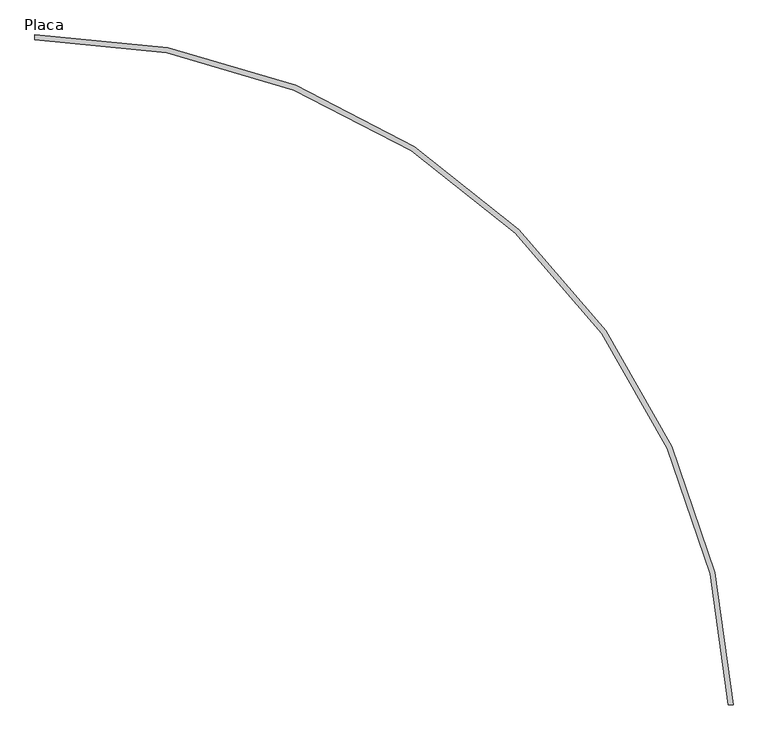
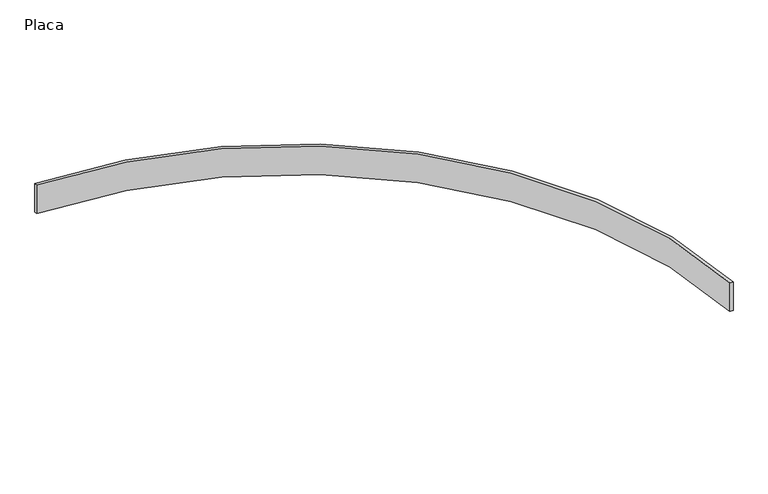
"""IFC4 building model written with IfcOpenShell, lengths in millimetres: beam geometry, Placa : banzo."""

from ifc_helpers import new_model, si_unit, point, frame, frame_2d, origin, place, context, project, spatial, polyline, circle_curve, trimmed, segment, composite_curve, outline, extrude, source, transform, mapped, element, save


def placa_baf9a1a6(model_context):
    return source(origin(), model_context, "Body", "SweptSolid", [
        extrude(outline(composite_curve([segment(polyline([(2241.2218755, -2143.1619319), (2225.2353227, -2143.8177733)]), True, "CONTINUOUS"), segment(trimmed(circle_curve(frame_2d((0.0, -2235.1070877)), 2227.1070877), [point((2225.2353227, -2143.8177733))], [point((0.0, -8.0))], True, "CARTESIAN"), True, "CONTINUOUS"), segment(polyline([(0.0, -8.0), (0.0, 8.0)]), True, "CONTINUOUS"), segment(trimmed(circle_curve(frame_2d((0.0, -2235.1070877)), 2243.1070877), [point((0.0, 8.0))], [point((2241.2218755, -2143.1619319))], False, "CARTESIAN"), True, "CONTINUOUS")], self_intersect=False)), frame((0.0, 0.0, -75.0), z_axis=(0.0, 0.0, 1.0), x_axis=(1.0, 0.0, 0.0)), (0.0, 0.0, 1.0), 150.0),
    ])


if __name__ == "__main__":
    model = new_model("IFC4")
    model_context = context("Model", 3, world=origin())
    ifc_project = project(units=[si_unit("LENGTHUNIT", "METRE", prefix="MILLI")], contexts=[model_context])
    site = spatial("IfcSite", under=ifc_project)
    building = spatial("IfcBuilding", under=site)
    placement = place(None, origin())
    placa_shape = placa_baf9a1a6(model_context)
    element("IfcBeam", 1, ObjectType="Placa : banzo", at=placement, inside=building, context=model_context, shape_type="MappedRepresentation", body=[
        mapped(placa_shape, transform((0.0, 0.0, 0.0), x_axis=(1.0, 0.0, 0.0), y_axis=(0.0, 1.0, 0.0), z_axis=(0.0, 0.0, 1.0))),
    ])
    save(model, "model.ifc")

# Revit data of these elements
# Type "Placa : banzo"
#   W = 0
#   Length [instance default] = 1.50 m
#   b = 0.15 m
#   d = 0.016 m
#   A = 0 m²
#   Structural Material [instance default] = Aço, 45-345
# Element 1 (IfcBeam, "Placa : banzo")
#   Materials on its faces: "Aço, 45-345"
# Materials
#   "Aço, 45-345": class "Metal", colour RGB 247 247 247, transparency 0, Description = "Aço 345 MPa", Cost = 0
